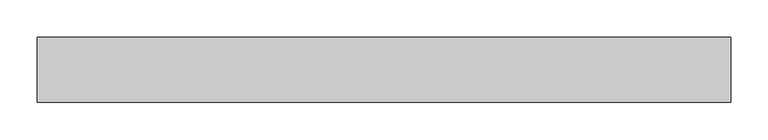
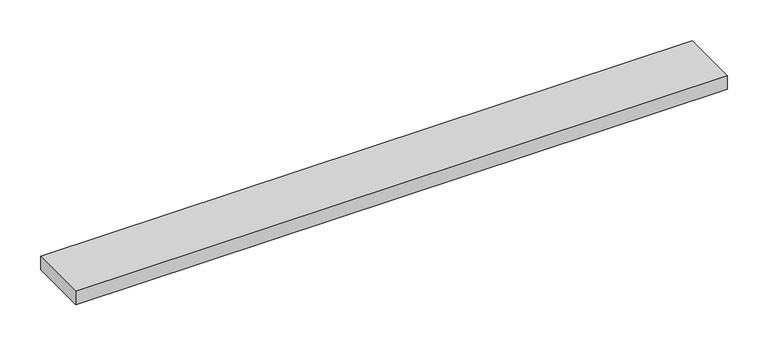
"""IFC4 building model written with IfcOpenShell, lengths in millimetres: proxy geometry, Generic Models 6:Generic Models 2:318829:Generic Models 2:318829 : Generic Models 6:Generic Models 2:318829:15 : Generic Models 6:Generic Models 2:318829:Generic Models 2:318829 : Generic Models 6:Generic Models 2:318829:300683."""

from ifc_helpers import new_model, si_unit, frame, origin, place, context, project, spatial, polyline, outline, extrude, source, transform, mapped, element, save


def generic_models_396ef59d(model_context):
    return source(origin(), model_context, "Body", "SweptSolid", [
        extrude(outline(polyline([(570394.5036635, -579003.173699), (570394.5036635, -579089.5913841), (569469.9742239, -579089.5913841), (569469.9742239, -579003.173699), (570394.5036635, -579003.173699)])), frame((0.0, 0.0, 2.841894), z_axis=(0.0, 0.0, 1.0), x_axis=(1.0, 0.0, 0.0)), (0.0, 0.0, 1.0), 20.3452501),
    ])


if __name__ == "__main__":
    model = new_model("IFC4")
    model_context = context("Model", 3, world=origin())
    ifc_project = project(units=[si_unit("LENGTHUNIT", "METRE", prefix="MILLI")], contexts=[model_context])
    site = spatial("IfcSite", under=ifc_project)
    building = spatial("IfcBuilding", under=site)
    placement = place(None, origin())
    generic_models_shape = generic_models_396ef59d(model_context)
    element("IfcBuildingElementProxy", 1, Name="Generic Models 6:Generic Models 2:318829:Generic Models 2:318829 : Generic Models 6:Generic Models 2:318829:15 : Generic Models 6:Generic Models 2:318829:Generic Models 2:318829 : Generic Models 6:Generic Models 2:318829:300683", ObjectType="Generic Models 6:Generic Models 2:318829:Generic Models 2:318829 : Generic Models 6:Generic Models 2:318829:15 : Generic Models 6:Generic Models 2:318829:Generic Models 2:318829 : Generic Models 6:Generic Models 2:318829:300683", at=placement, inside=building, context=model_context, shape_type="MappedRepresentation", body=[
        mapped(generic_models_shape, transform((0.0, 0.0, 0.0), x_axis=(1.0, 0.0, 0.0), y_axis=(0.0, 1.0, 0.0), z_axis=(0.0, 0.0, 1.0))),
    ])
    save(model, "model.ifc")

# Revit data of these elements
# Type "Generic Models 6:Generic Models 2:318829:Generic Models 2:318829 : Generic Models 6:Generic Models 2:318829:15 : Generic Models 6:Generic Models 2:318829:Generic Models 2:318829 : Generic Models 6:Generic Models 2:318829:300683"
#   NameOverride = "Generic Models 6:Generic Models 2:318829:Generic Models 2:318829 : Generic Models 6:Generic Models 2:318829:300683"
#   ObjectTypeOverride = "Generic Models 2:318829 : Generic Models 6:Generic Models 2:318829"
#   Reference = "Generic Models 2"
#   Tag = "300683"
# Element 1 (IfcBuildingElementProxy, "Generic Models 6:Generic Models 2:318829:Generic Models 2:318829 : Generic Models 6:Generic Models 2:318829:15 : Generic Models 6:Generic Models 2:318829:Generic Models 2:318829 : Generic Models 6:Generic Models 2:318829:300683")
#   Materials on its faces: "PRESSURE TREATED WOOD BLOCKING - SIZE AS NECESSARY"
# Materials
#   "PRESSURE TREATED WOOD BLOCKING - SIZE AS NECESSARY": class "Wood", colour RGB 144 113 62, transparency 0, Description = "Pinus Echinata", Cost = 0
